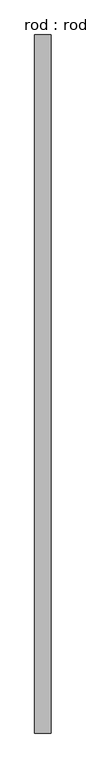
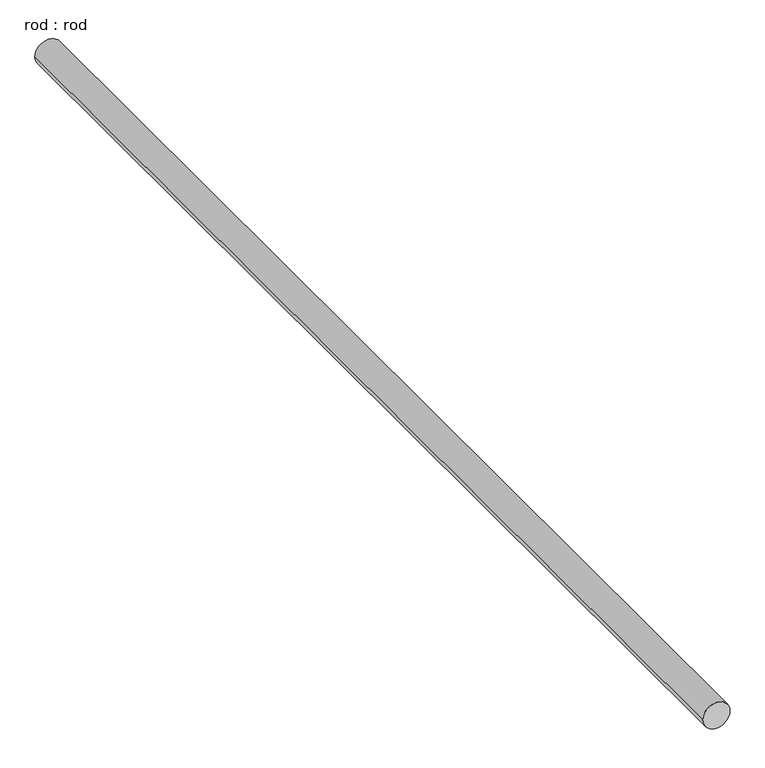
"""IFC4 building model written with IfcOpenShell, lengths in millimetres: proxy geometry, rod : rod."""

from ifc_helpers import new_model, si_unit, point, frame, frame_2d, origin, place, context, project, spatial, circle_curve, trimmed, segment, composite_curve, outline, extrude, source, transform, mapped, element, save


def rod_rod_1d80788d(model_context):
    return source(origin(), model_context, "Body", "SweptSolid", [
        extrude(outline(composite_curve([segment(trimmed(circle_curve(frame_2d((0.0108462, 0.0)), 200.0), [point((0.0108462, 200.0))], [point((0.0108462, -200.0))], False, "CARTESIAN"), True, "CONTINUOUS"), segment(trimmed(circle_curve(frame_2d((0.0108462, 0.0)), 200.0), [point((0.0108462, -200.0))], [point((0.0108462, 200.0))], False, "CARTESIAN"), True, "CONTINUOUS")], self_intersect=False)), frame((0.0, -4442.9856704, 0.0), z_axis=(0.0, 1.0, 0.0), x_axis=(0.0, 0.0, 1.0)), (0.0, 0.0, 1.0), 17071.4285714),
    ])


if __name__ == "__main__":
    model = new_model("IFC4")
    model_context = context("Model", 3, world=origin())
    ifc_project = project(units=[si_unit("LENGTHUNIT", "METRE", prefix="MILLI")], contexts=[model_context])
    site = spatial("IfcSite", under=ifc_project)
    building = spatial("IfcBuilding", under=site)
    placement = place(None, origin())
    rod_rod_shape = rod_rod_1d80788d(model_context)
    element("IfcBuildingElementProxy", 1, Name="rod : rod", ObjectType="rod : rod", at=placement, inside=building, context=model_context, shape_type="MappedRepresentation", body=[
        mapped(rod_rod_shape, transform((0.0, 0.0, 0.0), x_axis=(1.0, 0.0, 0.0), y_axis=(0.0, 1.0, 0.0), z_axis=(0.0, 0.0, 1.0))),
    ])
    save(model, "model.ifc")

# Revit data of these elements
# Type "rod : rod"
#   Default Elevation = 0
